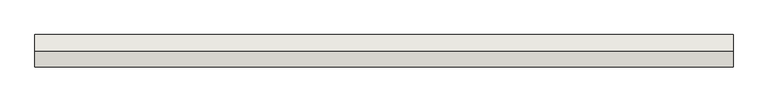
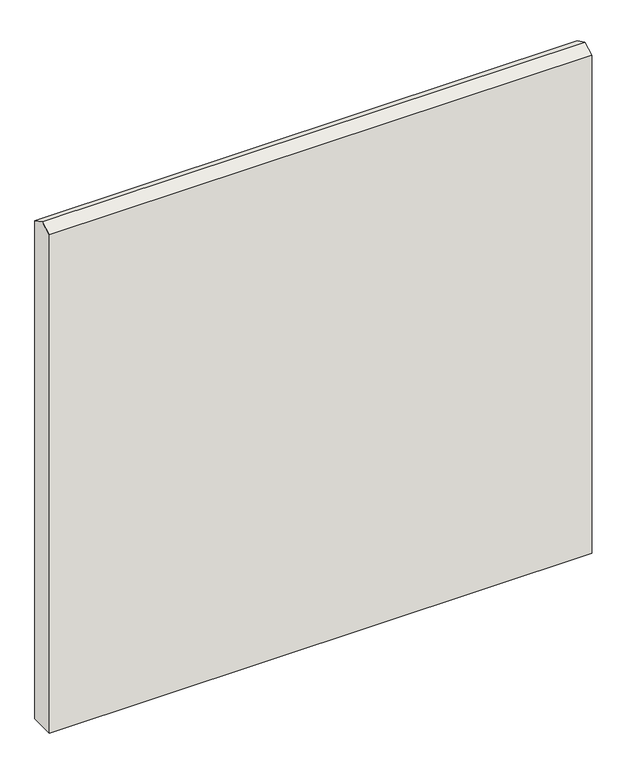
"""IFC4 building model written with IfcOpenShell, lengths in millimetres: wall geometry, Holzwand."""

from ifc_helpers import new_model, si_unit, frame, origin, place, context, project, spatial, polyline, outline, extrude, source, transform, mapped, element, save


def wall_50fd2b1e(model_context):
    return source(origin(), model_context, "Body", "SweptSolid", [
        extrude(outline(polyline([(100.0, 4251.6781465), (200.0, 4200.7256015), (200.0, 0.0), (0.0, 0.0), (0.0, 4200.7256015), (100.0, 4251.6781465)])), frame((0.0, 0.0, 0.0), z_axis=(1.0, 0.0, 0.0), x_axis=(0.0, 1.0, 0.0)), (0.0, 0.0, 1.0), 4327.8619019),
    ])


if __name__ == "__main__":
    model = new_model("IFC4")
    model_context = context("Model", 3, world=origin())
    ifc_project = project(units=[si_unit("LENGTHUNIT", "METRE", prefix="MILLI")], contexts=[model_context])
    site = spatial("IfcSite", under=ifc_project)
    building = spatial("IfcBuilding", under=site)
    placement = place(None, origin())
    wall_shape = wall_50fd2b1e(model_context)
    element("IfcWall", 1, ObjectType="Holzwand", at=placement, inside=building, context=model_context, shape_type="MappedRepresentation", body=[
        mapped(wall_shape, transform((0.0, 0.0, 0.0), x_axis=(1.0, 0.0, 0.0), y_axis=(0.0, 1.0, 0.0), z_axis=(0.0, 0.0, 1.0))),
    ])
    save(model, "model.ifc")

# Revit data of these elements
# Element 1 (IfcWall, "Holzwand")
#   Materials on its faces: "holzschalung"
# Materials
#   "holzschalung": class "Unassigned", colour RGB 128 128 128, transparency 0
